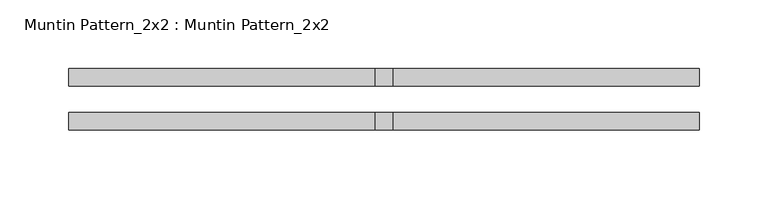
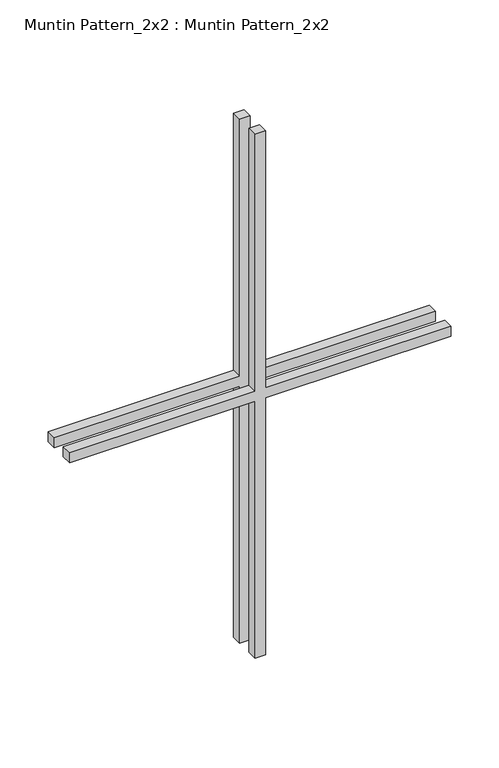
"""IFC4 building model written with IfcOpenShell, lengths in millimetres: proxy geometry, Muntin Pattern_2x2 : Muntin Pattern_2x2."""

from ifc_helpers import new_model, si_unit, frame, origin, place, context, project, spatial, polyline, outline, extrude, source, transform, mapped, element, save


def muntin_pattern_2x2_muntin_pattern_2x2_10aeb893(model_context):
    return source(origin(), model_context, "Body", "SweptSolid", [
        extrude(outline(polyline([(338.1375, -6.35), (338.1375, -228.6), (325.4375, -228.6), (325.4375, -6.35), (0.0, -6.35), (0.0, 6.35), (325.4375, 6.35), (325.4375, 228.6), (338.1375, 228.6), (338.1375, 6.35), (663.575, 6.35), (663.575, -6.35), (338.1375, -6.35)])), frame((0.0, -22.225, 0.0), z_axis=(0.0, 1.0, 0.0), x_axis=(0.0, 0.0, 1.0)), (0.0, 0.0, 1.0), 12.7),
        extrude(outline(polyline([(338.1375, -6.35), (338.1375, -228.6), (325.4375, -228.6), (325.4375, -6.35), (0.0, -6.35), (0.0, 6.35), (325.4375, 6.35), (325.4375, 228.6), (338.1375, 228.6), (338.1375, 6.35), (663.575, 6.35), (663.575, -6.35), (338.1375, -6.35)])), frame((0.0, 9.525, 0.0), z_axis=(0.0, 1.0, 0.0), x_axis=(0.0, 0.0, 1.0)), (0.0, 0.0, 1.0), 12.7),
    ])


if __name__ == "__main__":
    model = new_model("IFC4")
    model_context = context("Model", 3, world=origin())
    ifc_project = project(units=[si_unit("LENGTHUNIT", "METRE", prefix="MILLI")], contexts=[model_context])
    site = spatial("IfcSite", under=ifc_project)
    building = spatial("IfcBuilding", under=site)
    placement = place(None, origin())
    muntin_pattern_2x2_muntin_pattern_2x2_shape = muntin_pattern_2x2_muntin_pattern_2x2_10aeb893(model_context)
    element("IfcBuildingElementProxy", 1, Name="Muntin Pattern_2x2 : Muntin Pattern_2x2", ObjectType="Muntin Pattern_2x2 : Muntin Pattern_2x2", at=placement, inside=building, context=model_context, shape_type="MappedRepresentation", body=[
        mapped(muntin_pattern_2x2_muntin_pattern_2x2_shape, transform((0.0, 0.0, 0.0), x_axis=(1.0, 0.0, 0.0), y_axis=(0.0, 1.0, 0.0), z_axis=(0.0, 0.0, 1.0))),
    ])
    save(model, "model.ifc")

# Revit data of these elements
# Type "Muntin Pattern_2x2 : Muntin Pattern_2x2"
#   Width [instance default] = 4' - 0"
#   Thickness = 0' - 0 1/2"
#   Height [instance default] = 4' - 0"
#   Distance = 0' - 0 3/4"
#   Interior Material [instance default] = none
#   Exterior Material [instance default] = none
#   Default Elevation = 0
# Element 1 (IfcBuildingElementProxy, "Muntin Pattern_2x2 : Muntin Pattern_2x2")
#   Width = 1' - 6"
#   Height = 2' - 2 1/8"
#   Interior Material = Wood - Stained
#   Exterior Material = Clad - White
#   Materials on its faces: "Clad - White", "Wood - Stained"
# Materials
#   "Clad - White": class "Wood", colour RGB 242 242 238, transparency 0, Cost = 0
#   "Wood - Stained": class "Wood", colour RGB 224 178 126, transparency 0, Cost = 0
